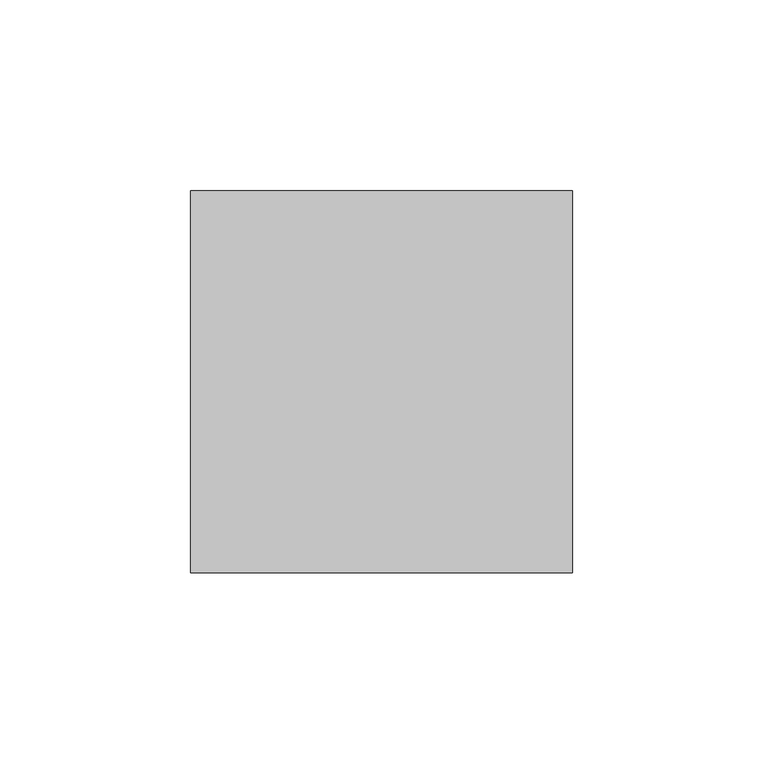
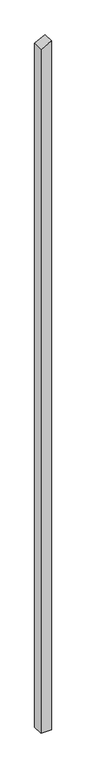
"""IFC4 building model written with IfcOpenShell, lengths in millimetres: column geometry, Holzstütze 160156 : Holzstütze 160156."""

from ifc_helpers import new_model, si_unit, frame, origin, place, context, project, spatial, polyline, outline, extrude, source, transform, mapped, element, save


def column_d24b82d5(model_context):
    return source(origin(), model_context, "Body", "SweptSolid", [
        extrude(outline(polyline([(-500.0, 157297.7593015), (-500.0, 157397.7593015), (6396.6643707, 157397.7593015), (6345.7118258, 157297.7593015), (-500.0, 157297.7593015)])), frame((0.0, 26981.9343946, 0.0), z_axis=(0.0, 1.0, 0.0), x_axis=(0.0, 0.0, 1.0)), (0.0, 0.0, 1.0), 100.0),
    ])


if __name__ == "__main__":
    model = new_model("IFC4")
    model_context = context("Model", 3, world=origin())
    ifc_project = project(units=[si_unit("LENGTHUNIT", "METRE", prefix="MILLI")], contexts=[model_context])
    site = spatial("IfcSite", under=ifc_project)
    building = spatial("IfcBuilding", under=site)
    placement = place(None, origin())
    column_shape = column_d24b82d5(model_context)
    element("IfcColumn", 1, ObjectType="Holzstütze 160156 : Holzstütze 160156", at=placement, inside=building, context=model_context, shape_type="MappedRepresentation", body=[
        mapped(column_shape, transform((0.0, 0.0, 0.0), x_axis=(1.0, 0.0, 0.0), y_axis=(0.0, 1.0, 0.0), z_axis=(0.0, 0.0, 1.0))),
    ])
    save(model, "model.ifc")

# Revit data of these elements
# Type "Holzstütze 160156 : Holzstütze 160156"
#   Abrechnungsart = "m"
#   Allright_Bauteil_ID = "0152St 0000143350"
#   Bezeichnung = "Holzstütze"
#   Codetext = "ST-HOLZ\\"
#   Gewerk = "Zimmer- und Holzbauarbeiten"
#   Material = "Holz"
#   Objektname = "Stütze"
#   NameOverride = "Holzstütze"
#   Reference = "Holzstütze"
#   Status = "NEW"
#   ThermalTransmittance = 0.0000 BTU/(h·ft²·°F)
#   Roll = 0.00°
#   Slope = 0.00°
#   2D Interaktion = yes
#   IsExternal = yes
#   LoadBearing = yes
# Element 1 (IfcColumn, "Holzstütze 160156 : Holzstütze 160156")
#   Materials on its faces: "holzschalung"
# Materials
#   "holzschalung": class "Unassigned", colour RGB 128 128 128, transparency 0
